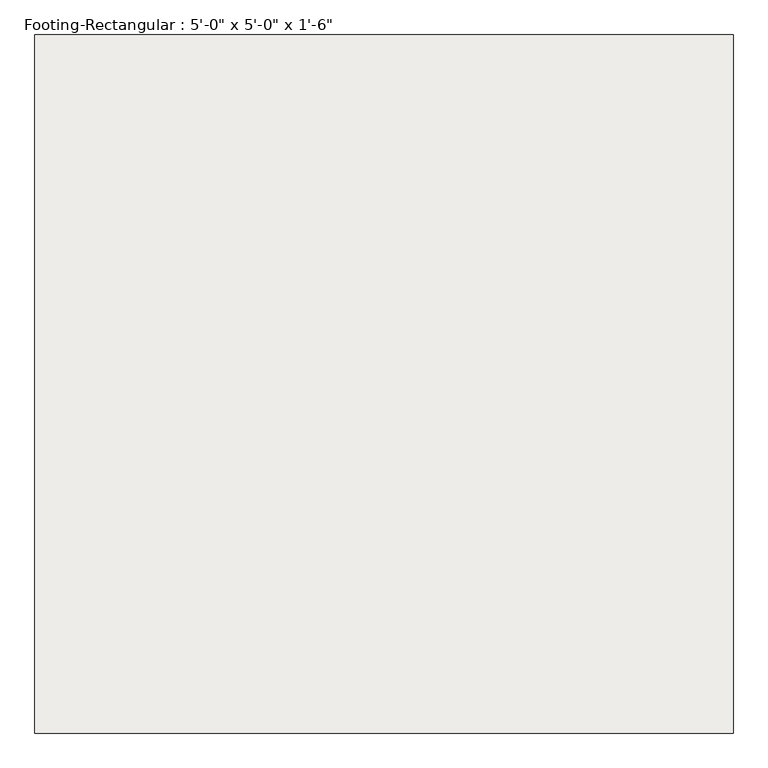
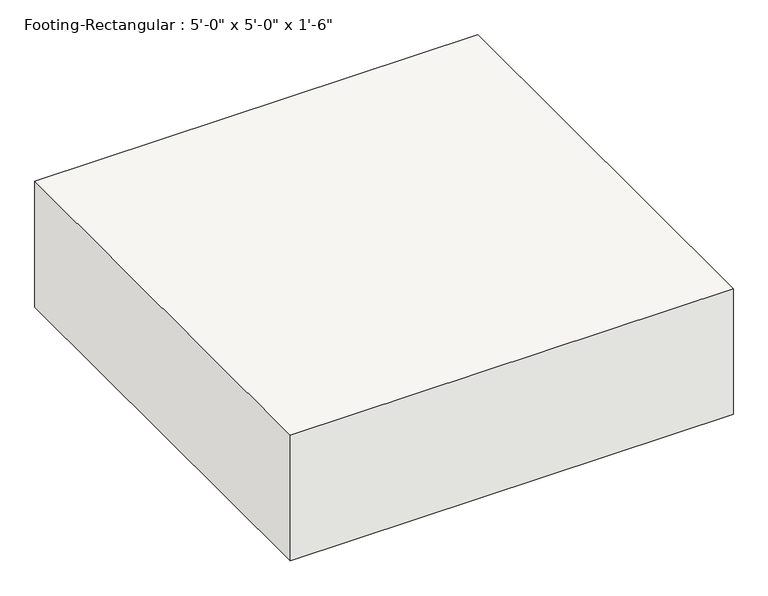
"""IFC4 building model written with IfcOpenShell, lengths in millimetres: slab geometry."""

from ifc_helpers import new_model, si_unit, frame, origin, place, context, project, spatial, polyline, outline, extrude, source, transform, mapped, element, save


def slab_df1ede25(model_context):
    return source(origin(), model_context, "Body", "SweptSolid", [
        extrude(outline(polyline([(762.0, 762.0), (762.0, -762.0), (-762.0, -762.0), (-762.0, 762.0), (762.0, 762.0)])), frame((0.0, 0.0, -457.2), z_axis=(0.0, 0.0, 1.0), x_axis=(1.0, 0.0, 0.0)), (0.0, 0.0, 1.0), 457.2),
    ])


if __name__ == "__main__":
    model = new_model("IFC4")
    model_context = context("Model", 3, world=origin())
    ifc_project = project(units=[si_unit("LENGTHUNIT", "METRE", prefix="MILLI")], contexts=[model_context])
    site = spatial("IfcSite", under=ifc_project)
    building = spatial("IfcBuilding", under=site)
    placement = place(None, origin())
    slab_shape = slab_df1ede25(model_context)
    element("IfcSlab", 1, ObjectType="Footing-Rectangular : 5'-0\" x 5'-0\" x 1'-6\"", at=placement, inside=building, context=model_context, shape_type="MappedRepresentation", body=[
        mapped(slab_shape, transform((0.0, 0.0, 0.0), x_axis=(1.0, 0.0, 0.0), y_axis=(0.0, 1.0, 0.0), z_axis=(0.0, 0.0, 1.0))),
    ])
    save(model, "model.ifc")

# Revit data of these elements
# Type "Footing-Rectangular : 5'-0\" x 5'-0\" x 1'-6\""
#   Description = ""
#   Assembly Code = "A1010100"
#   Width = 1524 mm
#   Length = 1524 mm
#   Thickness = 457.2 mm
#   Structural Material [instance default] = Concrete, Cast-in-Place gray
# Element 1 (IfcSlab, "Footing-Rectangular : 5'-0\" x 5'-0\" x 1'-6\"")
#   Materials on its faces: "Concrete, Cast-in-Place gray"
# Materials
#   "Concrete, Cast-in-Place gray": class "Concrete", colour RGB 192 192 192, transparency 0, Description = "Cast-in-place concrete", Cost = 0
